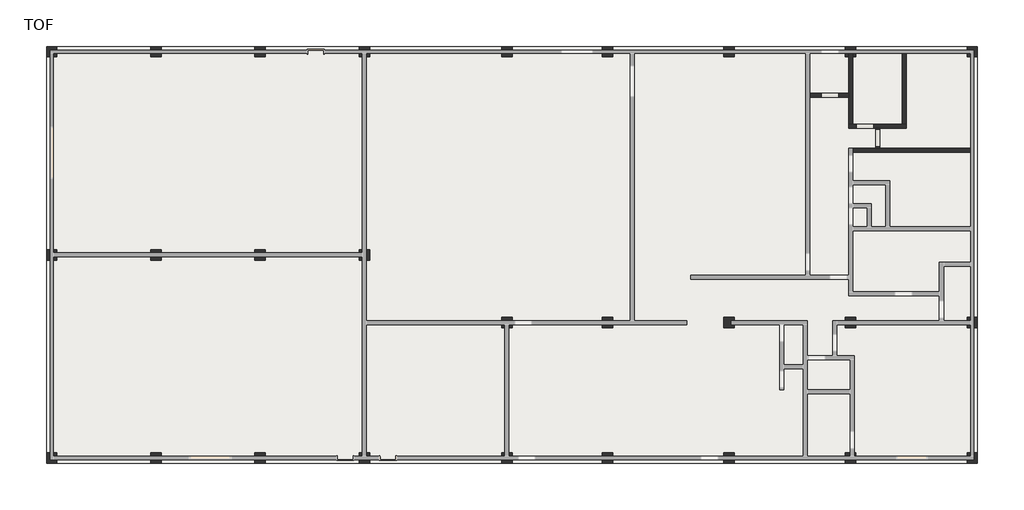
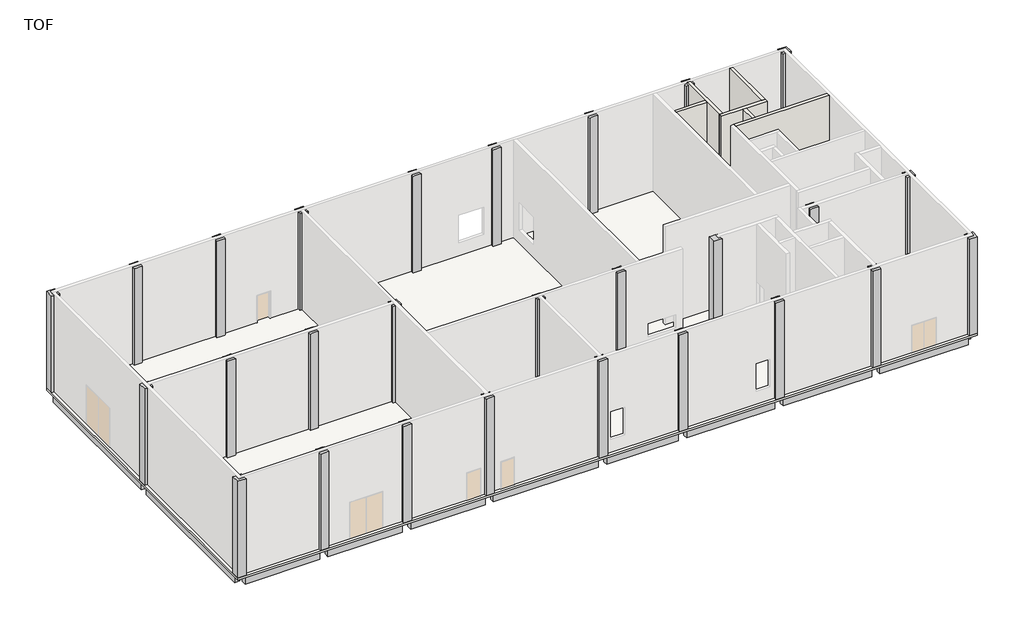
# One storey, part 2 of 2: 27 columns, 20 beams, 6 walls, 1 slab.
"""IFC4 building model written with IfcOpenShell, lengths in millimetres."""

from ifc_helpers import new_model, si_unit, frame, origin, place, context, project, spatial, polyline, outline, extrude, faceted_brep, element, save

model = new_model("IFC4")

# Units and contexts
model_context = context("Model", 3, world=origin())
ifc_project = project(units=[si_unit("LENGTHUNIT", "METRE", prefix="MILLI")], contexts=[model_context])

# Site, building, storey
site = spatial("IfcSite", under=ifc_project)
building = spatial("IfcBuilding", under=site)
storey = spatial("IfcBuildingStorey", under=building, Name="TOF", Elevation=149.9618634)

# Beams
placement = place(None, origin())
element("IfcBeam", 1, ObjectType="RC Beam_Rectangular : H_SB_AR_S16_TG_B400xH600", at=placement, inside=storey, context=model_context, shape_type="SweptSolid", body=[
    extrude(outline(polyline([(52825.0, 23599.5208589), (53175.0, 23599.5208589), (53175.0, 8599.5208589), (52825.0, 8599.5208589), (52825.0, 23599.5208589)])), frame((0.0, 0.0, -600.0), z_axis=(0.0, 0.0, 1.0), x_axis=(1.0, 0.0, 0.0)), (0.0, 0.0, 1.0), 600.0),
])
element("IfcBeam", 2, ObjectType="RC Beam_Rectangular : H_SB_AR_S16_TG_B400xH600", at=placement, inside=storey, context=model_context, shape_type="SweptSolid", body=[
    extrude(outline(polyline([(52825.0, 7999.5208589), (53175.0, 7999.5208589), (53175.0, 799.5208589), (52825.0, 799.5208589), (52825.0, 7999.5208589)])), frame((0.0, 0.0, -600.0), z_axis=(0.0, 0.0, 1.0), x_axis=(1.0, 0.0, 0.0)), (0.0, 0.0, 1.0), 600.0),
])
element("IfcBeam", 3, ObjectType="RC Beam_Rectangular : H_SB_AR_S16_TG_B400xH600", at=placement, inside=storey, context=model_context, shape_type="SweptSolid", body=[
    extrude(outline(polyline([(175.0, 12499.5208589), (-175.0, 12499.5208589), (-175.0, 23599.5208589), (175.0, 23599.5208589), (175.0, 12499.5208589)])), frame((0.0, 0.0, -600.0), z_axis=(0.0, 0.0, 1.0), x_axis=(1.0, 0.0, 0.0)), (0.0, 0.0, 1.0), 600.0),
])
element("IfcBeam", 4, ObjectType="RC Beam_Rectangular : H_SB_AR_S16_TG_B400xH600", at=placement, inside=storey, context=model_context, shape_type="SweptSolid", body=[
    extrude(outline(polyline([(-175.0, 11899.5208589), (175.0, 11899.5208589), (175.0, 799.5208589), (-175.0, 799.5208589), (-175.0, 11899.5208589)])), frame((0.0, 0.0, -600.0), z_axis=(0.0, 0.0, 1.0), x_axis=(1.0, 0.0, 0.0)), (0.0, 0.0, 1.0), 600.0),
])
element("IfcBeam", 5, ObjectType="RC Beam_Rectangular : H_SB_AR_S16_TG_B400xH600", at=placement, inside=storey, context=model_context, shape_type="SweptSolid", body=[
    extrude(outline(polyline([(300.0, 23724.5208589), (300.0, 24074.5208589), (5700.0, 24074.5208589), (5700.0, 23724.5208589), (300.0, 23724.5208589)])), frame((0.0, 0.0, -600.0), z_axis=(0.0, 0.0, 1.0), x_axis=(1.0, 0.0, 0.0)), (0.0, 0.0, 1.0), 600.0),
])
element("IfcBeam", 6, ObjectType="RC Beam_Rectangular : H_SB_AR_S16_TG_B400xH600", at=placement, inside=storey, context=model_context, shape_type="SweptSolid", body=[
    extrude(outline(polyline([(6300.0, 23724.5208589), (6300.0, 24074.5208589), (11700.0, 24074.5208589), (11700.0, 23724.5208589), (6300.0, 23724.5208589)])), frame((0.0, 0.0, -600.0), z_axis=(0.0, 0.0, 1.0), x_axis=(1.0, 0.0, 0.0)), (0.0, 0.0, 1.0), 600.0),
])
element("IfcBeam", 7, ObjectType="RC Beam_Rectangular : H_SB_AR_S16_TG_B400xH600", at=placement, inside=storey, context=model_context, shape_type="SweptSolid", body=[
    extrude(outline(polyline([(12300.0, 23724.5208589), (12300.0, 24074.5208589), (17700.0, 24074.5208589), (17700.0, 23724.5208589), (12300.0, 23724.5208589)])), frame((0.0, 0.0, -600.0), z_axis=(0.0, 0.0, 1.0), x_axis=(1.0, 0.0, 0.0)), (0.0, 0.0, 1.0), 600.0),
])
element("IfcBeam", 8, ObjectType="RC Beam_Rectangular : H_SB_AR_S16_TG_B400xH600", at=placement, inside=storey, context=model_context, shape_type="SweptSolid", body=[
    extrude(outline(polyline([(18300.0, 23724.5208589), (18300.0, 24074.5208589), (25900.0, 24074.5208589), (25900.0, 23724.5208589), (18300.0, 23724.5208589)])), frame((0.0, 0.0, -600.0), z_axis=(0.0, 0.0, 1.0), x_axis=(1.0, 0.0, 0.0)), (0.0, 0.0, 1.0), 600.0),
])
element("IfcBeam", 9, ObjectType="RC Beam_Rectangular : H_SB_AR_S16_TG_B400xH600", at=placement, inside=storey, context=model_context, shape_type="SweptSolid", body=[
    extrude(outline(polyline([(26500.0, 23724.5208589), (26500.0, 24074.5208589), (31700.0, 24074.5208589), (31700.0, 23724.5208589), (26500.0, 23724.5208589)])), frame((0.0, 0.0, -600.0), z_axis=(0.0, 0.0, 1.0), x_axis=(1.0, 0.0, 0.0)), (0.0, 0.0, 1.0), 600.0),
])
element("IfcBeam", 10, ObjectType="RC Beam_Rectangular : H_SB_AR_S16_TG_B400xH600", at=placement, inside=storey, context=model_context, shape_type="SweptSolid", body=[
    extrude(outline(polyline([(32300.0, 23724.5208589), (32300.0, 24074.5208589), (38700.0, 24074.5208589), (38700.0, 23724.5208589), (32300.0, 23724.5208589)])), frame((0.0, 0.0, -600.0), z_axis=(0.0, 0.0, 1.0), x_axis=(1.0, 0.0, 0.0)), (0.0, 0.0, 1.0), 600.0),
])
element("IfcBeam", 11, ObjectType="RC Beam_Rectangular : H_SB_AR_S16_TG_B400xH600", at=placement, inside=storey, context=model_context, shape_type="SweptSolid", body=[
    extrude(outline(polyline([(39300.0, 23724.5208589), (39300.0, 24074.5208589), (45700.0, 24074.5208589), (45700.0, 23724.5208589), (39300.0, 23724.5208589)])), frame((0.0, 0.0, -600.0), z_axis=(0.0, 0.0, 1.0), x_axis=(1.0, 0.0, 0.0)), (0.0, 0.0, 1.0), 600.0),
])
element("IfcBeam", 12, ObjectType="RC Beam_Rectangular : H_SB_AR_S16_TG_B400xH600", at=placement, inside=storey, context=model_context, shape_type="SweptSolid", body=[
    extrude(outline(polyline([(52700.0, 24074.5208589), (52700.0, 23724.5208589), (46300.0, 23724.5208589), (46300.0, 24074.5208589), (52700.0, 24074.5208589)])), frame((0.0, 0.0, -600.0), z_axis=(0.0, 0.0, 1.0), x_axis=(1.0, 0.0, 0.0)), (0.0, 0.0, 1.0), 600.0),
])
element("IfcBeam", 13, ObjectType="RC Beam_Rectangular : H_SB_AR_S16_TG_B400xH600", at=placement, inside=storey, context=model_context, shape_type="SweptSolid", body=[
    extrude(outline(polyline([(300.0, 324.5208589), (300.0, 674.5208589), (5700.0, 674.5208589), (5700.0, 324.5208589), (300.0, 324.5208589)])), frame((0.0, 0.0, -600.0), z_axis=(0.0, 0.0, 1.0), x_axis=(1.0, 0.0, 0.0)), (0.0, 0.0, 1.0), 600.0),
])
element("IfcBeam", 14, ObjectType="RC Beam_Rectangular : H_SB_AR_S16_TG_B400xH600", at=placement, inside=storey, context=model_context, shape_type="SweptSolid", body=[
    extrude(outline(polyline([(6300.0, 324.5208589), (6300.0, 674.5208589), (11700.0, 674.5208589), (11700.0, 324.5208589), (6300.0, 324.5208589)])), frame((0.0, 0.0, -600.0), z_axis=(0.0, 0.0, 1.0), x_axis=(1.0, 0.0, 0.0)), (0.0, 0.0, 1.0), 600.0),
])
element("IfcBeam", 15, ObjectType="RC Beam_Rectangular : H_SB_AR_S16_TG_B400xH600", at=placement, inside=storey, context=model_context, shape_type="SweptSolid", body=[
    extrude(outline(polyline([(12300.0, 324.5208589), (12300.0, 674.5208589), (17700.0, 674.5208589), (17700.0, 324.5208589), (12300.0, 324.5208589)])), frame((0.0, 0.0, -600.0), z_axis=(0.0, 0.0, 1.0), x_axis=(1.0, 0.0, 0.0)), (0.0, 0.0, 1.0), 600.0),
])
element("IfcBeam", 16, ObjectType="RC Beam_Rectangular : H_SB_AR_S16_TG_B400xH600", at=placement, inside=storey, context=model_context, shape_type="SweptSolid", body=[
    extrude(outline(polyline([(18300.0, 324.5208589), (18300.0, 674.5208589), (25900.0, 674.5208589), (25900.0, 324.5208589), (18300.0, 324.5208589)])), frame((0.0, 0.0, -600.0), z_axis=(0.0, 0.0, 1.0), x_axis=(1.0, 0.0, 0.0)), (0.0, 0.0, 1.0), 600.0),
])
element("IfcBeam", 17, ObjectType="RC Beam_Rectangular : H_SB_AR_S16_TG_B400xH600", at=placement, inside=storey, context=model_context, shape_type="SweptSolid", body=[
    extrude(outline(polyline([(26500.0, 324.5208589), (26500.0, 674.5208589), (31700.0, 674.5208589), (31700.0, 324.5208589), (26500.0, 324.5208589)])), frame((0.0, 0.0, -600.0), z_axis=(0.0, 0.0, 1.0), x_axis=(1.0, 0.0, 0.0)), (0.0, 0.0, 1.0), 600.0),
])
element("IfcBeam", 18, ObjectType="RC Beam_Rectangular : H_SB_AR_S16_TG_B400xH600", at=placement, inside=storey, context=model_context, shape_type="SweptSolid", body=[
    extrude(outline(polyline([(32300.0, 324.5208589), (32300.0, 674.5208589), (38700.0, 674.5208589), (38700.0, 324.5208589), (32300.0, 324.5208589)])), frame((0.0, 0.0, -600.0), z_axis=(0.0, 0.0, 1.0), x_axis=(1.0, 0.0, 0.0)), (0.0, 0.0, 1.0), 600.0),
])
element("IfcBeam", 19, ObjectType="RC Beam_Rectangular : H_SB_AR_S16_TG_B400xH600", at=placement, inside=storey, context=model_context, shape_type="SweptSolid", body=[
    extrude(outline(polyline([(39300.0, 324.5208589), (39300.0, 674.5208589), (45700.0, 674.5208589), (45700.0, 324.5208589), (39300.0, 324.5208589)])), frame((0.0, 0.0, -600.0), z_axis=(0.0, 0.0, 1.0), x_axis=(1.0, 0.0, 0.0)), (0.0, 0.0, 1.0), 600.0),
])
element("IfcBeam", 20, ObjectType="RC Beam_Rectangular : H_SB_AR_S16_TG_B400xH600", at=placement, inside=storey, context=model_context, shape_type="SweptSolid", body=[
    extrude(outline(polyline([(52700.0, 674.5208589), (52700.0, 324.5208589), (46300.0, 324.5208589), (46300.0, 674.5208589), (52700.0, 674.5208589)])), frame((0.0, 0.0, -600.0), z_axis=(0.0, 0.0, 1.0), x_axis=(1.0, 0.0, 0.0)), (0.0, 0.0, 1.0), 600.0),
])

# Columns
element("IfcColumn", 21, ObjectType="RC_Column_Rectangular : H_SC_AR_S15_W600xL600", at=placement, inside=storey, context=model_context, shape_type="Brep", body=[
    faceted_brep([(300.0, 12499.5208589, 149.9618634), (300.0, 11899.5208589, 149.9618634), (-300.0, 11899.5208589, 149.9618634), (-300.0, 12499.5208589, 149.9618634), (300.0, 12499.5208589, 7548.9618634), (300.0, 12349.5208589, 7548.9618634), (300.0, 12049.5208589, 7548.9618634), (300.0, 11899.5208589, 7548.9618634), (150.0, 11899.5208589, 7548.9618634), (-150.0, 11899.5208589, 7548.9618634), (-300.0, 11899.5208589, 7548.9618634), (-300.0, 12499.5208589, 7548.9618634), (-150.0, 12499.5208589, 7548.9618634), (150.0, 12499.5208589, 7548.9618634)], [[[0, 1, 2, 3]], [[1, 0, 4, 5, 6, 7]], [[2, 1, 7, 8, 9, 10]], [[3, 2, 10, 11]], [[0, 3, 11, 12, 13, 4]], [[7, 6, 5, 4, 13, 12, 11, 10, 9, 8]]]),
])
element("IfcColumn", 22, ObjectType="RC_Column_Rectangular : H_SC_AR_S15_W600xL600", at=placement, inside=storey, context=model_context, shape_type="Brep", body=[
    faceted_brep([(6300.0, 12499.5208589, 149.9618634), (6300.0, 11899.5208589, 149.9618634), (5700.0, 11899.5208589, 149.9618634), (5700.0, 12499.5208589, 149.9618634), (6300.0, 12499.5208589, 7548.9618634), (6300.0, 12349.5208589, 7548.9618634), (6300.0, 12049.5208589, 7548.9618634), (6300.0, 11899.5208589, 7548.9618634), (6150.0, 11899.5208589, 7548.9618634), (5850.0, 11899.5208589, 7548.9618634), (5700.0, 11899.5208589, 7548.9618634), (5700.0, 12049.5208589, 7548.9618634), (5700.0, 12349.5208589, 7548.9618634), (5700.0, 12499.5208589, 7548.9618634), (5850.0, 12499.5208589, 7548.9618634), (6150.0, 12499.5208589, 7548.9618634)], [[[0, 1, 2, 3]], [[1, 0, 4, 5, 6, 7]], [[2, 1, 7, 8, 9, 10]], [[3, 2, 10, 11, 12, 13]], [[0, 3, 13, 14, 15, 4]], [[7, 6, 5, 4, 15, 14, 13, 12, 11, 10, 9, 8]]]),
])
element("IfcColumn", 23, ObjectType="RC_Column_Rectangular : H_SC_AR_S15_W600xL600", at=placement, inside=storey, context=model_context, shape_type="Brep", body=[
    faceted_brep([(12300.0, 12499.5208589, 149.9618634), (12300.0, 11899.5208589, 149.9618634), (11700.0, 11899.5208589, 149.9618634), (11700.0, 12499.5208589, 149.9618634), (12300.0, 12499.5208589, 7548.9618634), (12300.0, 12349.5208589, 7548.9618634), (12300.0, 12049.5208589, 7548.9618634), (12300.0, 11899.5208589, 7548.9618634), (12150.0, 11899.5208589, 7548.9618634), (11850.0, 11899.5208589, 7548.9618634), (11700.0, 11899.5208589, 7548.9618634), (11700.0, 12049.5208589, 7548.9618634), (11700.0, 12349.5208589, 7548.9618634), (11700.0, 12499.5208589, 7548.9618634), (11850.0, 12499.5208589, 7548.9618634), (12150.0, 12499.5208589, 7548.9618634)], [[[0, 1, 2, 3]], [[1, 0, 4, 5, 6, 7]], [[2, 1, 7, 8, 9, 10]], [[3, 2, 10, 11, 12, 13]], [[0, 3, 13, 14, 15, 4]], [[7, 6, 5, 4, 15, 14, 13, 12, 11, 10, 9, 8]]]),
])
element("IfcColumn", 24, ObjectType="RC_Column_Rectangular : H_SC_AR_S15_W600xL600", at=placement, inside=storey, context=model_context, shape_type="Brep", body=[
    faceted_brep([(18300.0, 12499.5208589, 149.9618634), (18300.0, 11899.5208589, 149.9618634), (17700.0, 11899.5208589, 149.9618634), (17700.0, 12499.5208589, 149.9618634), (18300.0, 12499.5208589, 7548.9618634), (18300.0, 11899.5208589, 7548.9618634), (18150.0, 11899.5208589, 7548.9618634), (17850.0, 11899.5208589, 7548.9618634), (17700.0, 11899.5208589, 7548.9618634), (17700.0, 12049.5208589, 7548.9618634), (17700.0, 12349.5208589, 7548.9618634), (17700.0, 12499.5208589, 7548.9618634), (17850.0, 12499.5208589, 7548.9618634), (18150.0, 12499.5208589, 7548.9618634)], [[[0, 1, 2, 3]], [[1, 0, 4, 5]], [[2, 1, 5, 6, 7, 8]], [[3, 2, 8, 9, 10, 11]], [[0, 3, 11, 12, 13, 4]], [[5, 4, 13, 12, 11, 10, 9, 8, 7, 6]]]),
])
element("IfcColumn", 25, ObjectType="RC_Column_Rectangular : H_SC_AR_S15_W600xL600", at=placement, inside=storey, context=model_context, shape_type="Brep", body=[
    faceted_brep([(300.0, 24199.5208589, 149.9618634), (300.0, 23599.5208589, 149.9618634), (-300.0, 23599.5208589, 149.9618634), (-300.0, 24199.5208589, 149.9618634), (300.0, 24199.5208589, 7548.9618634), (300.0, 24049.5208589, 7548.9618634), (300.0, 23749.5208589, 7548.9618634), (300.0, 23599.5208589, 7548.9618634), (150.0, 23599.5208589, 7548.9618634), (-150.0, 23599.5208589, 7548.9618634), (-300.0, 23599.5208589, 7548.9618634), (-300.0, 24199.5208589, 7548.9618634)], [[[0, 1, 2, 3]], [[1, 0, 4, 5, 6, 7]], [[2, 1, 7, 8, 9, 10]], [[3, 2, 10, 11]], [[0, 3, 11, 4]], [[7, 6, 5, 4, 11, 10, 9, 8]]]),
])
element("IfcColumn", 26, ObjectType="RC_Column_Rectangular : H_SC_AR_S15_W600xL600", at=placement, inside=storey, context=model_context, shape_type="Brep", body=[
    faceted_brep([(6300.0, 24199.5208589, 149.9618634), (6300.0, 23599.5208589, 149.9618634), (5700.0, 23599.5208589, 149.9618634), (5700.0, 24199.5208589, 149.9618634), (6300.0, 24199.5208589, 7548.9618634), (6300.0, 24049.5208589, 7548.9618634), (6300.0, 23749.5208589, 7548.9618634), (6300.0, 23599.5208589, 7548.9618634), (6150.0, 23599.5208589, 7548.9618634), (5850.0, 23599.5208589, 7548.9618634), (5700.0, 23599.5208589, 7548.9618634), (5700.0, 23749.5208589, 7548.9618634), (5700.0, 24049.5208589, 7548.9618634), (5700.0, 24199.5208589, 7548.9618634)], [[[0, 1, 2, 3]], [[1, 0, 4, 5, 6, 7]], [[2, 1, 7, 8, 9, 10]], [[3, 2, 10, 11, 12, 13]], [[0, 3, 13, 4]], [[7, 6, 5, 4, 13, 12, 11, 10, 9, 8]]]),
])
element("IfcColumn", 27, ObjectType="RC_Column_Rectangular : H_SC_AR_S15_W600xL600", at=placement, inside=storey, context=model_context, shape_type="Brep", body=[
    faceted_brep([(12300.0, 24199.5208589, 149.9618634), (12300.0, 23599.5208589, 149.9618634), (11700.0, 23599.5208589, 149.9618634), (11700.0, 24199.5208589, 149.9618634), (12300.0, 24199.5208589, 7548.9618634), (12300.0, 24049.5208589, 7548.9618634), (12300.0, 23749.5208589, 7548.9618634), (12300.0, 23599.5208589, 7548.9618634), (12150.0, 23599.5208589, 7548.9618634), (11850.0, 23599.5208589, 7548.9618634), (11700.0, 23599.5208589, 7548.9618634), (11700.0, 23749.5208589, 7548.9618634), (11700.0, 24049.5208589, 7548.9618634), (11700.0, 24199.5208589, 7548.9618634)], [[[0, 1, 2, 3]], [[1, 0, 4, 5, 6, 7]], [[2, 1, 7, 8, 9, 10]], [[3, 2, 10, 11, 12, 13]], [[0, 3, 13, 4]], [[7, 6, 5, 4, 13, 12, 11, 10, 9, 8]]]),
])
element("IfcColumn", 28, ObjectType="RC_Column_Rectangular : H_SC_AR_S15_W600xL600", at=placement, inside=storey, context=model_context, shape_type="Brep", body=[
    faceted_brep([(18300.0, 24199.5208589, 149.9618634), (18300.0, 23599.5208589, 149.9618634), (17700.0, 23599.5208589, 149.9618634), (17700.0, 24199.5208589, 149.9618634), (18300.0, 24199.5208589, 7548.9618634), (18300.0, 24049.5208589, 7548.9618634), (18300.0, 23749.5208589, 7548.9618634), (18300.0, 23599.5208589, 7548.9618634), (18150.0, 23599.5208589, 7548.9618634), (17850.0, 23599.5208589, 7548.9618634), (17700.0, 23599.5208589, 7548.9618634), (17700.0, 23749.5208589, 7548.9618634), (17700.0, 24049.5208589, 7548.9618634), (17700.0, 24199.5208589, 7548.9618634)], [[[0, 1, 2, 3]], [[1, 0, 4, 5, 6, 7]], [[2, 1, 7, 8, 9, 10]], [[3, 2, 10, 11, 12, 13]], [[0, 3, 13, 4]], [[7, 6, 5, 4, 13, 12, 11, 10, 9, 8]]]),
])
element("IfcColumn", 29, ObjectType="RC_Column_Rectangular : H_SC_AR_S15_W600xL600", at=placement, inside=storey, context=model_context, shape_type="Brep", body=[
    faceted_brep([(26500.0, 24199.5208589, 149.9618634), (26500.0, 23599.5208589, 149.9618634), (25900.0, 23599.5208589, 149.9618634), (25900.0, 24199.5208589, 149.9618634), (26500.0, 24199.5208589, 7548.9618634), (26500.0, 24049.5208589, 7548.9618634), (26500.0, 23749.5208589, 7548.9618634), (26500.0, 23599.5208589, 7548.9618634), (26350.0, 23599.5208589, 7548.9618634), (26050.0, 23599.5208589, 7548.9618634), (25900.0, 23599.5208589, 7548.9618634), (25900.0, 23749.5208589, 7548.9618634), (25900.0, 24049.5208589, 7548.9618634), (25900.0, 24199.5208589, 7548.9618634)], [[[0, 1, 2, 3]], [[1, 0, 4, 5, 6, 7]], [[2, 1, 7, 8, 9, 10]], [[3, 2, 10, 11, 12, 13]], [[0, 3, 13, 4]], [[7, 6, 5, 4, 13, 12, 11, 10, 9, 8]]]),
])
element("IfcColumn", 30, ObjectType="RC_Column_Rectangular : H_SC_AR_S15_W600xL600", at=placement, inside=storey, context=model_context, shape_type="Brep", body=[
    faceted_brep([(32300.0, 24199.5208589, 149.9618634), (32300.0, 23599.5208589, 149.9618634), (31700.0, 23599.5208589, 149.9618634), (31700.0, 24199.5208589, 149.9618634), (32300.0, 24199.5208589, 7548.9618634), (32300.0, 24049.5208589, 7548.9618634), (32300.0, 23749.5208589, 7548.9618634), (32300.0, 23599.5208589, 7548.9618634), (32150.0, 23599.5208589, 7548.9618634), (31850.0, 23599.5208589, 7548.9618634), (31700.0, 23599.5208589, 7548.9618634), (31700.0, 23749.5208589, 7548.9618634), (31700.0, 24049.5208589, 7548.9618634), (31700.0, 24199.5208589, 7548.9618634)], [[[0, 1, 2, 3]], [[1, 0, 4, 5, 6, 7]], [[2, 1, 7, 8, 9, 10]], [[3, 2, 10, 11, 12, 13]], [[0, 3, 13, 4]], [[7, 6, 5, 4, 13, 12, 11, 10, 9, 8]]]),
])
element("IfcColumn", 31, ObjectType="RC_Column_Rectangular : H_SC_AR_S15_W600xL600", at=placement, inside=storey, context=model_context, shape_type="Brep", body=[
    faceted_brep([(39300.0, 24199.5208589, 149.9618634), (39300.0, 23599.5208589, 149.9618634), (38700.0, 23599.5208589, 149.9618634), (38700.0, 24199.5208589, 149.9618634), (39300.0, 24199.5208589, 7548.9618634), (39300.0, 24049.5208589, 7548.9618634), (39300.0, 23749.5208589, 7548.9618634), (39300.0, 23599.5208589, 7548.9618634), (39150.0, 23599.5208589, 7548.9618634), (38850.0, 23599.5208589, 7548.9618634), (38700.0, 23599.5208589, 7548.9618634), (38700.0, 23749.5208589, 7548.9618634), (38700.0, 24049.5208589, 7548.9618634), (38700.0, 24199.5208589, 7548.9618634)], [[[0, 1, 2, 3]], [[1, 0, 4, 5, 6, 7]], [[2, 1, 7, 8, 9, 10]], [[3, 2, 10, 11, 12, 13]], [[0, 3, 13, 4]], [[7, 6, 5, 4, 13, 12, 11, 10, 9, 8]]]),
])
element("IfcColumn", 32, ObjectType="RC_Column_Rectangular : H_SC_AR_S15_W600xL600", at=placement, inside=storey, context=model_context, shape_type="Brep", body=[
    faceted_brep([(46300.0, 24199.5208589, 149.9618634), (46300.0, 23599.5208589, 149.9618634), (45700.0, 23599.5208589, 149.9618634), (45700.0, 24199.5208589, 149.9618634), (46300.0, 24199.5208589, 7548.9618634), (46300.0, 24049.5208589, 7548.9618634), (46300.0, 23749.5208589, 7548.9618634), (46300.0, 23599.5208589, 7548.9618634), (46150.0, 23599.5208589, 7548.9618634), (45850.0, 23599.5208589, 7548.9618634), (45700.0, 23599.5208589, 7548.9618634), (45700.0, 23749.5208589, 7548.9618634), (45700.0, 24049.5208589, 7548.9618634), (45700.0, 24199.5208589, 7548.9618634)], [[[0, 1, 2, 3]], [[1, 0, 4, 5, 6, 7]], [[2, 1, 7, 8, 9, 10]], [[3, 2, 10, 11, 12, 13]], [[0, 3, 13, 4]], [[7, 6, 5, 4, 13, 12, 11, 10, 9, 8]]]),
])
element("IfcColumn", 33, ObjectType="RC_Column_Rectangular : H_SC_AR_S15_W600xL600", at=placement, inside=storey, context=model_context, shape_type="Brep", body=[
    faceted_brep([(53300.0, 24199.5208589, 149.9618634), (53300.0, 23599.5208589, 149.9618634), (52700.0, 23599.5208589, 149.9618634), (52700.0, 24199.5208589, 149.9618634), (53300.0, 24199.5208589, 7548.9618634), (53300.0, 23599.5208589, 7548.9618634), (53150.0, 23599.5208589, 7548.9618634), (52850.0, 23599.5208589, 7548.9618634), (52700.0, 23599.5208589, 7548.9618634), (52700.0, 23749.5208589, 7548.9618634), (52700.0, 24049.5208589, 7548.9618634), (52700.0, 24199.5208589, 7548.9618634)], [[[0, 1, 2, 3]], [[1, 0, 4, 5]], [[2, 1, 5, 6, 7, 8]], [[3, 2, 8, 9, 10, 11]], [[0, 3, 11, 4]], [[5, 4, 11, 10, 9, 8, 7, 6]]]),
])
element("IfcColumn", 34, ObjectType="RC_Column_Rectangular : H_SC_AR_S15_W600xL600", at=placement, inside=storey, context=model_context, shape_type="Brep", body=[
    faceted_brep([(26500.0, 8599.5208589, 149.9618634), (26500.0, 7999.5208589, 149.9618634), (25900.0, 7999.5208589, 149.9618634), (25900.0, 8599.5208589, 149.9618634), (26500.0, 8599.5208589, 7548.9618634), (26500.0, 8449.5208589, 7548.9618634), (26500.0, 8149.5208589, 7548.9618634), (26500.0, 7999.5208589, 7548.9618634), (26350.0, 7999.5208589, 7548.9618634), (26050.0, 7999.5208589, 7548.9618634), (25900.0, 7999.5208589, 7548.9618634), (25900.0, 8599.5208589, 7548.9618634), (26050.0, 8599.5208589, 7548.9618634), (26350.0, 8599.5208589, 7548.9618634)], [[[0, 1, 2, 3]], [[1, 0, 4, 5, 6, 7]], [[2, 1, 7, 8, 9, 10]], [[3, 2, 10, 11]], [[0, 3, 11, 12, 13, 4]], [[7, 6, 5, 4, 13, 12, 11, 10, 9, 8]]]),
])
element("IfcColumn", 35, ObjectType="RC_Column_Rectangular : H_SC_AR_S15_W600xL600", at=placement, inside=storey, context=model_context, shape_type="Brep", body=[
    faceted_brep([(32300.0, 8599.5208589, 149.9618634), (32300.0, 7999.5208589, 149.9618634), (31700.0, 7999.5208589, 149.9618634), (31700.0, 8599.5208589, 149.9618634), (32300.0, 8599.5208589, 7548.9618634), (32300.0, 8449.5208589, 7548.9618634), (32300.0, 8149.5208589, 7548.9618634), (32300.0, 7999.5208589, 7548.9618634), (32150.0, 7999.5208589, 7548.9618634), (31850.0, 7999.5208589, 7548.9618634), (31700.0, 7999.5208589, 7548.9618634), (31700.0, 8149.5208589, 7548.9618634), (31700.0, 8449.5208589, 7548.9618634), (31700.0, 8599.5208589, 7548.9618634), (31850.0, 8599.5208589, 7548.9618634), (32150.0, 8599.5208589, 7548.9618634)], [[[0, 1, 2, 3]], [[1, 0, 4, 5, 6, 7]], [[2, 1, 7, 8, 9, 10]], [[3, 2, 10, 11, 12, 13]], [[0, 3, 13, 14, 15, 4]], [[7, 6, 5, 4, 15, 14, 13, 12, 11, 10, 9, 8]]]),
])
element("IfcColumn", 36, ObjectType="RC_Column_Rectangular : H_SC_AR_S15_W600xL600", at=placement, inside=storey, context=model_context, shape_type="Brep", body=[
    faceted_brep([(39300.0, 8599.5208589, 149.9618634), (39300.0, 7999.5208589, 149.9618634), (38700.0, 7999.5208589, 149.9618634), (38700.0, 8599.5208589, 149.9618634), (39300.0, 8599.5208589, 7548.9618634), (39300.0, 8449.5208589, 7548.9618634), (39300.0, 8149.5208589, 7548.9618634), (39300.0, 7999.5208589, 7548.9618634), (39150.0, 7999.5208589, 7548.9618634), (38850.0, 7999.5208589, 7548.9618634), (38700.0, 7999.5208589, 7548.9618634), (38700.0, 8149.5208589, 7548.9618634), (38700.0, 8449.5208589, 7548.9618634), (38700.0, 8599.5208589, 7548.9618634), (38850.0, 8599.5208589, 7548.9618634), (39150.0, 8599.5208589, 7548.9618634)], [[[0, 1, 2, 3]], [[1, 0, 4, 5, 6, 7]], [[2, 1, 7, 8, 9, 10]], [[3, 2, 10, 11, 12, 13]], [[0, 3, 13, 14, 15, 4]], [[7, 6, 5, 4, 15, 14, 13, 12, 11, 10, 9, 8]]]),
])
element("IfcColumn", 37, ObjectType="RC_Column_Rectangular : H_SC_AR_S15_W600xL600", at=placement, inside=storey, context=model_context, shape_type="Brep", body=[
    faceted_brep([(46300.0, 8599.5208589, 149.9618634), (46300.0, 7999.5208589, 149.9618634), (45700.0, 7999.5208589, 149.9618634), (45700.0, 8599.5208589, 149.9618634), (46300.0, 8599.5208589, 7548.9618634), (46300.0, 8449.5208589, 7548.9618634), (46300.0, 8149.5208589, 7548.9618634), (46300.0, 7999.5208589, 7548.9618634), (46150.0, 7999.5208589, 7548.9618634), (45850.0, 7999.5208589, 7548.9618634), (45700.0, 7999.5208589, 7548.9618634), (45700.0, 8149.5208589, 7548.9618634), (45700.0, 8449.5208589, 7548.9618634), (45700.0, 8599.5208589, 7548.9618634), (45850.0, 8599.5208589, 7548.9618634), (46150.0, 8599.5208589, 7548.9618634)], [[[0, 1, 2, 3]], [[1, 0, 4, 5, 6, 7]], [[2, 1, 7, 8, 9, 10]], [[3, 2, 10, 11, 12, 13]], [[0, 3, 13, 14, 15, 4]], [[7, 6, 5, 4, 15, 14, 13, 12, 11, 10, 9, 8]]]),
])
element("IfcColumn", 38, ObjectType="RC_Column_Rectangular : H_SC_AR_S15_W600xL600", at=placement, inside=storey, context=model_context, shape_type="Brep", body=[
    faceted_brep([(53300.0, 8599.5208589, 149.9618634), (53300.0, 7999.5208589, 149.9618634), (52700.0, 7999.5208589, 149.9618634), (52700.0, 8599.5208589, 149.9618634), (53300.0, 8599.5208589, 7548.9618634), (53300.0, 7999.5208589, 7548.9618634), (53150.0, 7999.5208589, 7548.9618634), (52850.0, 7999.5208589, 7548.9618634), (52700.0, 7999.5208589, 7548.9618634), (52700.0, 8149.5208589, 7548.9618634), (52700.0, 8449.5208589, 7548.9618634), (52700.0, 8599.5208589, 7548.9618634), (52850.0, 8599.5208589, 7548.9618634), (53150.0, 8599.5208589, 7548.9618634)], [[[0, 1, 2, 3]], [[1, 0, 4, 5]], [[2, 1, 5, 6, 7, 8]], [[3, 2, 8, 9, 10, 11]], [[0, 3, 11, 12, 13, 4]], [[5, 4, 13, 12, 11, 10, 9, 8, 7, 6]]]),
])
element("IfcColumn", 39, ObjectType="RC_Column_Rectangular : H_SC_AR_S15_W600xL600", at=placement, inside=storey, context=model_context, shape_type="Brep", body=[
    faceted_brep([(300.0, 799.5208589, 149.9618634), (300.0, 199.5208589, 149.9618634), (-300.0, 199.5208589, 149.9618634), (-300.0, 799.5208589, 149.9618634), (300.0, 799.5208589, 7548.9618634), (300.0, 649.5208589, 7548.9618634), (300.0, 349.5208589, 7548.9618634), (300.0, 199.5208589, 7548.9618634), (-300.0, 199.5208589, 7548.9618634), (-300.0, 799.5208589, 7548.9618634), (-150.0, 799.5208589, 7548.9618634), (150.0, 799.5208589, 7548.9618634)], [[[0, 1, 2, 3]], [[1, 0, 4, 5, 6, 7]], [[2, 1, 7, 8]], [[3, 2, 8, 9]], [[0, 3, 9, 10, 11, 4]], [[7, 6, 5, 4, 11, 10, 9, 8]]]),
])
element("IfcColumn", 40, ObjectType="RC_Column_Rectangular : H_SC_AR_S15_W600xL600", at=placement, inside=storey, context=model_context, shape_type="Brep", body=[
    faceted_brep([(6300.0, 799.5208589, 149.9618634), (6300.0, 199.5208589, 149.9618634), (5700.0, 199.5208589, 149.9618634), (5700.0, 799.5208589, 149.9618634), (6300.0, 799.5208589, 7548.9618634), (6300.0, 649.5208589, 7548.9618634), (6300.0, 349.5208589, 7548.9618634), (6300.0, 199.5208589, 7548.9618634), (5700.0, 199.5208589, 7548.9618634), (5700.0, 349.5208589, 7548.9618634), (5700.0, 649.5208589, 7548.9618634), (5700.0, 799.5208589, 7548.9618634), (5850.0, 799.5208589, 7548.9618634), (6150.0, 799.5208589, 7548.9618634)], [[[0, 1, 2, 3]], [[1, 0, 4, 5, 6, 7]], [[2, 1, 7, 8]], [[3, 2, 8, 9, 10, 11]], [[0, 3, 11, 12, 13, 4]], [[7, 6, 5, 4, 13, 12, 11, 10, 9, 8]]]),
])
element("IfcColumn", 41, ObjectType="RC_Column_Rectangular : H_SC_AR_S15_W600xL600", at=placement, inside=storey, context=model_context, shape_type="Brep", body=[
    faceted_brep([(12300.0, 799.5208589, 149.9618634), (12300.0, 199.5208589, 149.9618634), (11700.0, 199.5208589, 149.9618634), (11700.0, 799.5208589, 149.9618634), (12300.0, 799.5208589, 7548.9618634), (12300.0, 649.5208589, 7548.9618634), (12300.0, 349.5208589, 7548.9618634), (12300.0, 199.5208589, 7548.9618634), (11700.0, 199.5208589, 7548.9618634), (11700.0, 349.5208589, 7548.9618634), (11700.0, 649.5208589, 7548.9618634), (11700.0, 799.5208589, 7548.9618634), (11850.0, 799.5208589, 7548.9618634), (12150.0, 799.5208589, 7548.9618634)], [[[0, 1, 2, 3]], [[1, 0, 4, 5, 6, 7]], [[2, 1, 7, 8]], [[3, 2, 8, 9, 10, 11]], [[0, 3, 11, 12, 13, 4]], [[7, 6, 5, 4, 13, 12, 11, 10, 9, 8]]]),
])
element("IfcColumn", 42, ObjectType="RC_Column_Rectangular : H_SC_AR_S15_W600xL600", at=placement, inside=storey, context=model_context, shape_type="Brep", body=[
    faceted_brep([(18300.0, 799.5208589, 149.9618634), (18300.0, 199.5208589, 149.9618634), (17700.0, 199.5208589, 149.9618634), (17700.0, 799.5208589, 149.9618634), (18300.0, 799.5208589, 7548.9618634), (18300.0, 649.5208589, 7548.9618634), (18300.0, 349.5208589, 7548.9618634), (18300.0, 199.5208589, 7548.9618634), (17700.0, 199.5208589, 7548.9618634), (17700.0, 349.5208589, 7548.9618634), (17700.0, 649.5208589, 7548.9618634), (17700.0, 799.5208589, 7548.9618634), (17850.0, 799.5208589, 7548.9618634), (18150.0, 799.5208589, 7548.9618634)], [[[0, 1, 2, 3]], [[1, 0, 4, 5, 6, 7]], [[2, 1, 7, 8]], [[3, 2, 8, 9, 10, 11]], [[0, 3, 11, 12, 13, 4]], [[7, 6, 5, 4, 13, 12, 11, 10, 9, 8]]]),
])
element("IfcColumn", 43, ObjectType="RC_Column_Rectangular : H_SC_AR_S15_W600xL600", at=placement, inside=storey, context=model_context, shape_type="Brep", body=[
    faceted_brep([(26500.0, 799.5208589, 149.9618634), (26500.0, 199.5208589, 149.9618634), (25900.0, 199.5208589, 149.9618634), (25900.0, 799.5208589, 149.9618634), (26500.0, 799.5208589, 7548.9618634), (26500.0, 649.5208589, 7548.9618634), (26500.0, 349.5208589, 7548.9618634), (26500.0, 199.5208589, 7548.9618634), (25900.0, 199.5208589, 7548.9618634), (25900.0, 349.5208589, 7548.9618634), (25900.0, 649.5208589, 7548.9618634), (25900.0, 799.5208589, 7548.9618634), (26050.0, 799.5208589, 7548.9618634), (26350.0, 799.5208589, 7548.9618634)], [[[0, 1, 2, 3]], [[1, 0, 4, 5, 6, 7]], [[2, 1, 7, 8]], [[3, 2, 8, 9, 10, 11]], [[0, 3, 11, 12, 13, 4]], [[7, 6, 5, 4, 13, 12, 11, 10, 9, 8]]]),
])
element("IfcColumn", 44, ObjectType="RC_Column_Rectangular : H_SC_AR_S15_W600xL600", at=placement, inside=storey, context=model_context, shape_type="Brep", body=[
    faceted_brep([(32300.0, 799.5208589, 149.9618634), (32300.0, 199.5208589, 149.9618634), (31700.0, 199.5208589, 149.9618634), (31700.0, 799.5208589, 149.9618634), (32300.0, 799.5208589, 7548.9618634), (32300.0, 649.5208589, 7548.9618634), (32300.0, 349.5208589, 7548.9618634), (32300.0, 199.5208589, 7548.9618634), (31700.0, 199.5208589, 7548.9618634), (31700.0, 349.5208589, 7548.9618634), (31700.0, 649.5208589, 7548.9618634), (31700.0, 799.5208589, 7548.9618634), (31850.0, 799.5208589, 7548.9618634), (32150.0, 799.5208589, 7548.9618634)], [[[0, 1, 2, 3]], [[1, 0, 4, 5, 6, 7]], [[2, 1, 7, 8]], [[3, 2, 8, 9, 10, 11]], [[0, 3, 11, 12, 13, 4]], [[7, 6, 5, 4, 13, 12, 11, 10, 9, 8]]]),
])
element("IfcColumn", 45, ObjectType="RC_Column_Rectangular : H_SC_AR_S15_W600xL600", at=placement, inside=storey, context=model_context, shape_type="Brep", body=[
    faceted_brep([(39300.0, 799.5208589, 149.9618634), (39300.0, 199.5208589, 149.9618634), (38700.0, 199.5208589, 149.9618634), (38700.0, 799.5208589, 149.9618634), (39300.0, 799.5208589, 7548.9618634), (39300.0, 649.5208589, 7548.9618634), (39300.0, 349.5208589, 7548.9618634), (39300.0, 199.5208589, 7548.9618634), (38700.0, 199.5208589, 7548.9618634), (38700.0, 349.5208589, 7548.9618634), (38700.0, 649.5208589, 7548.9618634), (38700.0, 799.5208589, 7548.9618634), (38850.0, 799.5208589, 7548.9618634), (39150.0, 799.5208589, 7548.9618634)], [[[0, 1, 2, 3]], [[1, 0, 4, 5, 6, 7]], [[2, 1, 7, 8]], [[3, 2, 8, 9, 10, 11]], [[0, 3, 11, 12, 13, 4]], [[7, 6, 5, 4, 13, 12, 11, 10, 9, 8]]]),
])
element("IfcColumn", 46, ObjectType="RC_Column_Rectangular : H_SC_AR_S15_W600xL600", at=placement, inside=storey, context=model_context, shape_type="Brep", body=[
    faceted_brep([(46300.0, 799.5208589, 149.9618634), (46300.0, 199.5208589, 149.9618634), (45700.0, 199.5208589, 149.9618634), (45700.0, 799.5208589, 149.9618634), (46300.0, 799.5208589, 7548.9618634), (46300.0, 649.5208589, 7548.9618634), (46300.0, 349.5208589, 7548.9618634), (46300.0, 199.5208589, 7548.9618634), (45700.0, 199.5208589, 7548.9618634), (45700.0, 349.5208589, 7548.9618634), (45700.0, 649.5208589, 7548.9618634), (45700.0, 799.5208589, 7548.9618634), (45850.0, 799.5208589, 7548.9618634), (46150.0, 799.5208589, 7548.9618634)], [[[0, 1, 2, 3]], [[1, 0, 4, 5, 6, 7]], [[2, 1, 7, 8]], [[3, 2, 8, 9, 10, 11]], [[0, 3, 11, 12, 13, 4]], [[7, 6, 5, 4, 13, 12, 11, 10, 9, 8]]]),
])
element("IfcColumn", 47, ObjectType="RC_Column_Rectangular : H_SC_AR_S15_W600xL600", at=placement, inside=storey, context=model_context, shape_type="Brep", body=[
    faceted_brep([(53300.0, 799.5208589, 149.9618634), (53300.0, 199.5208589, 149.9618634), (52700.0, 199.5208589, 149.9618634), (52700.0, 799.5208589, 149.9618634), (53300.0, 799.5208589, 7548.9618634), (53300.0, 199.5208589, 7548.9618634), (52700.0, 199.5208589, 7548.9618634), (52700.0, 349.5208589, 7548.9618634), (52700.0, 649.5208589, 7548.9618634), (52700.0, 799.5208589, 7548.9618634), (52850.0, 799.5208589, 7548.9618634), (53150.0, 799.5208589, 7548.9618634)], [[[0, 1, 2, 3]], [[1, 0, 4, 5]], [[2, 1, 5, 6]], [[3, 2, 6, 7, 8, 9]], [[0, 3, 9, 10, 11, 4]], [[5, 4, 11, 10, 9, 8, 7, 6]]]),
])

# Slab
element("IfcSlab", 48, ObjectType="H_FL_AR_S17_RC Slab T150", at=placement, inside=storey, context=model_context, shape_type="SweptSolid", body=[
    extrude(outline(polyline([(53300.0, 199.5208589), (-300.0, 199.5208589), (-300.0, 24199.5208589), (53300.0, 24199.5208589), (53300.0, 199.5208589)])), frame((0.0, 0.0, -0.0381366), z_axis=(0.0, 0.0, 1.0), x_axis=(1.0, 0.0, 0.0)), (0.0, 0.0, 1.0), 150.0),
])

# Walls
element("IfcWall", 49, ObjectType="H_WA_AR_B02_Int Wall_Block T200", at=placement, inside=storey, context=model_context, shape_type="SweptSolid", body=[
    extrude(outline(polyline([(149.9618634, 43647.0), (149.9618634, 45883.0), (7649.9618634, 45883.0), (7649.9618634, 43647.0), (149.9618634, 43647.0)]), holes=[polyline([(1149.9618634, 44300.0), (3249.9618634, 44300.0), (3249.9618634, 45300.0), (1149.9618634, 45300.0), (1149.9618634, 44300.0)])]), frame((0.0, 21277.5208589, 0.0), z_axis=(0.0, 1.0, 0.0), x_axis=(0.0, 0.0, 1.0)), (0.0, 0.0, 1.0), 234.0),
])
element("IfcWall", 50, ObjectType="H_WA_AR_B02_Int Wall_Block T200", at=placement, inside=storey, context=model_context, shape_type="Brep", body=[
    faceted_brep([(46117.0, 18102.5208589, 149.9618634), (52900.0, 18102.5208589, 149.9618634), (52900.0, 18102.5208589, 7649.9618634), (46117.0, 18102.5208589, 7649.9618634), (46117.0, 18336.5208589, 149.9618634), (46117.0, 18336.5208589, 7649.9618634), (47453.0, 18336.5208589, 7649.9618634), (47687.0, 18336.5208589, 7649.9618634), (52900.0, 18336.5208589, 7649.9618634), (52900.0, 18336.5208589, 149.9618634), (47687.0, 18336.5208589, 149.9618634), (47453.0, 18336.5208589, 149.9618634)], [[[0, 1, 2, 3]], [[4, 5, 6, 7, 8, 9, 10, 11]], [[1, 0, 4, 11, 10, 9]], [[3, 2, 8, 7, 6, 5]], [[2, 1, 9, 8]], [[0, 3, 5, 4]]]),
])
element("IfcWall", 51, ObjectType="H_WA_AR_B02_Int Wall_Block T200", at=placement, inside=storey, context=model_context, shape_type="Brep", body=[
    faceted_brep([(45883.0, 19502.5208589, 149.9618634), (47453.0, 19502.5208589, 149.9618634), (47687.0, 19502.5208589, 149.9618634), (49197.0, 19502.5208589, 149.9618634), (49197.0, 19502.5208589, 7649.9618634), (47687.0, 19502.5208589, 7649.9618634), (47453.0, 19502.5208589, 7649.9618634), (45883.0, 19502.5208589, 7649.9618634), (47325.0, 19502.5208589, 1149.9618634), (46325.0, 19502.5208589, 1149.9618634), (46325.0, 19502.5208589, 3249.9618634), (47325.0, 19502.5208589, 3249.9618634), (45883.0, 19736.5208589, 149.9618634), (45883.0, 19736.5208589, 7649.9618634), (46117.0, 19736.5208589, 7649.9618634), (48963.0, 19736.5208589, 7649.9618634), (49197.0, 19736.5208589, 7649.9618634), (49197.0, 19736.5208589, 149.9618634), (48963.0, 19736.5208589, 149.9618634), (46117.0, 19736.5208589, 149.9618634), (47325.0, 19736.5208589, 1149.9618634), (47325.0, 19736.5208589, 3249.9618634), (46325.0, 19736.5208589, 3249.9618634), (46325.0, 19736.5208589, 1149.9618634)], [[[0, 1, 2, 3, 4, 5, 6, 7], [8, 9, 10, 11]], [[12, 13, 14, 15, 16, 17, 18, 19], [20, 21, 22, 23]], [[3, 2, 1, 0, 12, 19, 18, 17]], [[7, 6, 5, 4, 16, 15, 14, 13]], [[4, 3, 17, 16]], [[0, 7, 13, 12]], [[21, 20, 8, 11]], [[22, 21, 11, 10]], [[23, 22, 10, 9]], [[20, 23, 9, 8]]]),
])
element("IfcWall", 52, ObjectType="H_WA_AR_B02_Int Wall_Block T200", at=placement, inside=storey, context=model_context, shape_type="SweptSolid", body=[
    extrude(outline(polyline([(49197.0, 23799.5208589), (49197.0, 19736.5208589), (48963.0, 19736.5208589), (48963.0, 23799.5208589), (49197.0, 23799.5208589)])), frame((0.0, 0.0, 149.9618634), z_axis=(0.0, 0.0, 1.0), x_axis=(1.0, 0.0, 0.0)), (0.0, 0.0, 1.0), 7500.0),
])
element("IfcWall", 53, ObjectType="H_WA_AR_B02_Int Wall_Block T200", at=placement, inside=storey, context=model_context, shape_type="SweptSolid", body=[
    extrude(outline(polyline([(19502.5208589, 149.9618634), (18336.5208589, 149.9618634), (18336.5208589, 7649.9618634), (19502.5208589, 7649.9618634), (19502.5208589, 149.9618634)]), holes=[polyline([(18424.5208589, 1149.9618634), (19424.5208589, 1149.9618634), (19424.5208589, 3249.9618634), (18424.5208589, 3249.9618634), (18424.5208589, 1149.9618634)])]), frame((47453.0, 0.0, 0.0), z_axis=(1.0, 0.0, 0.0), x_axis=(0.0, 1.0, 0.0)), (0.0, 0.0, 1.0), 234.0),
])
element("IfcWall", 54, ObjectType="H_WA_AR_B02_Int Wall_Block T200", at=placement, inside=storey, context=model_context, shape_type="Brep", body=[
    faceted_brep([(46117.0, 19736.5208589, 149.9618634), (46117.0, 23799.5208589, 149.9618634), (46117.0, 23799.5208589, 7649.9618634), (46117.0, 19736.5208589, 7649.9618634), (45883.0, 19736.5208589, 149.9618634), (45883.0, 19736.5208589, 7649.9618634), (45883.0, 21277.5208589, 7649.9618634), (45883.0, 21511.5208589, 7649.9618634), (45883.0, 23799.5208589, 7649.9618634), (45883.0, 23799.5208589, 149.9618634), (45883.0, 21511.5208589, 149.9618634), (45883.0, 21277.5208589, 149.9618634)], [[[0, 1, 2, 3]], [[4, 5, 6, 7, 8, 9, 10, 11]], [[1, 0, 4, 11, 10, 9]], [[3, 2, 8, 7, 6, 5]], [[2, 1, 9, 8]], [[0, 3, 5, 4]]]),
])

save(model, "model.ifc")

# Revit data of these elements
# Type "RC Beam_Rectangular : H_SB_AR_S16_TG_B400xH600"
#   중앙부 하부근 = ""
#   중앙부 상부근 = ""
#   중앙부 보조근 = ""
#   중앙부 늑근 = ""
#   외단부 하부근 = ""
#   외단부 상부근 = ""
#   외단부 보조근 = ""
#   외단부 늑근 = ""
#   부호 = "TG2"
#   내단부 하부근 = ""
#   내단부 상부근 = ""
#   내단부 보조근 = ""
#   내단부 늑근 = ""
#   ALL 하부근 = "3-D20"
#   ALL 상부근 = "4-D20"
#   ALL 보조근 = ""
#   ALL 늑근 = "2-D10 @120"
#   Width = 350 mm
#   Height = 600 mm
#   Length [instance default] = 1524 mm
#   b = 350 mm
#   h = 600 mm
#   hec_material3 [instance default] = none
#   hec_material2 [instance default] = none
#   hec_material1 [instance default] = none
#   Structural Material [instance default] = none
#   Assembly Code = ""
# Type "RC_Column_Rectangular : H_SC_AR_S15_W600xL600"
#   Width = 600 mm
#   Length = 600 mm
#   hec_material3 [instance default] = none
#   hec_material2 [instance default] = none
#   hec_material1 [instance default] = none
#   Structural Material [instance default] = none
#   Description = (empty or 0)
# Type "H_FL_AR_S17_RC Slab T150"
#   Keynote = ""
#   Type Comments = ""
#   Description = ""
#   Function = 1
#   Layers, outside or top first: 150 mm no material (function 1)
# Type "H_WA_AR_B02_Int Wall_Block T200"
#   Type Comments = ""
#   Layers, outside or top first: 0 mm no material (function 100); 12 mm no material (function 2); 200 mm no material (function 1); 12 mm no material (function 2); 10 mm no material (function 5)
# Elements 1, 2, 3, 4, 5, 6, 7, 8, 9, 10, 11, 12, 13, 14, 15, 16, 17, 18, 19, 20 (IfcBeam, "RC Beam_Rectangular : H_SB_AR_S16_TG_B400xH600")
#   Comments = ""
#   hec_material3 = none
#   hec_material2 = none
#   hec_material1 = none
#   Structural Material = none
#   Phase Created = New Construction
# Elements 21, 22, 23, 24, 25, 26, 27, 28, 29, 30, 31, 32, 33, 34, 35, 36, 37, 38, 39, 40, 41, 42, 43, 44, 45, 46, 47 (IfcColumn, "RC_Column_Rectangular : H_SC_AR_S15_W600xL600")
#   Comments = ""
#   hec_material3 = none
#   hec_material2 = none
#   hec_material1 = none
#   Structural Material = none
#   Phase Created = New Construction
# Element 48 (IfcSlab, "H_FL_AR_S17_RC Slab T150")
#   Height Offset From Level = 0 mm
#   Phase Created = New Construction
#   Materials on its faces: "Default Floor"
# Elements 49, 50, 51, 52, 53, 54 (IfcWall, "H_WA_AR_B02_Int Wall_Block T200")
#   H_Wall Style Name = "Block Wall"
#   H_Wall-Base Material-1 = "Concrete Block"
#   H_Wall-Base Material-2 = ""
#   H_Wall_Finish-In = "Acrylic Emulsion Paint on Cement Plaster"
#   H_Wall_Base Material-3 = ""
#   H_Wall_Finish-Ex = "Acrylic Emulsion Paint on Cement Plaster"
#   H_Wall_Style Remark = "WM : Reinforced Concrete Block\n     50mm<THK≤100mm / 100mm<THK≤200mm / 200mm<THK"
#   Top Offset = 0 mm
#   Base Offset = 0 mm
#   wall height = 7500 mm
#   H_Wall Style No = IW21
#   Phase Created = New Construction
#   Base Constraint = TOF
#   Top Constraint = TOC
#   Materials on its faces: "Default Wall"
# Materials
#   "Default Floor": class "Miscellaneous", colour RGB 80 80 80, transparency 0
#   "Default Wall": class "Miscellaneous", colour RGB 80 80 80, transparency 0
